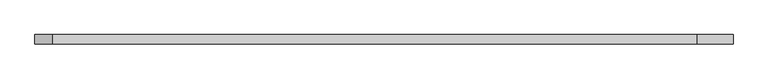
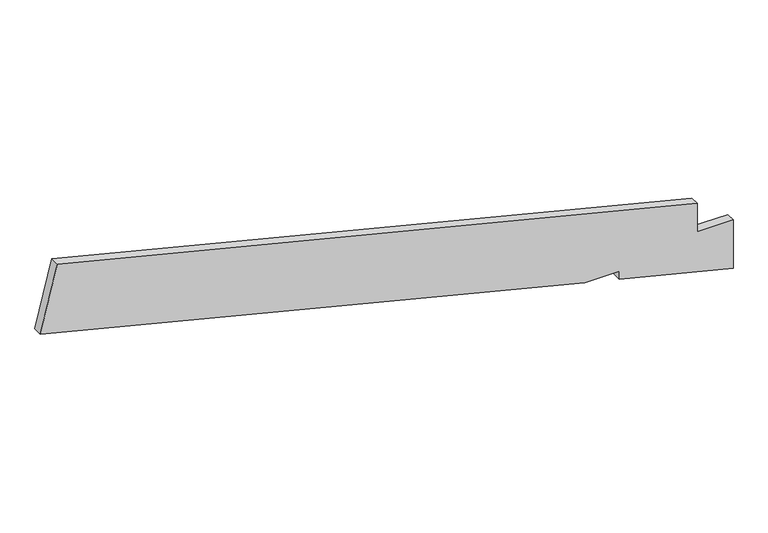
"""IFC4 building model written with IfcOpenShell, lengths in millimetres: proxy geometry, Generic Models 288:Generic Models 288:157157 : Generic Models 288:Generic Models 288:157157."""

from ifc_helpers import new_model, si_unit, frame, origin, place, context, project, spatial, polyline, outline, extrude, source, transform, mapped, element, save


def generic_models_c55f884c(model_context):
    return source(origin(), model_context, "Body", "SweptSolid", [
        extrude(outline(polyline([(6276.29133, 1895.353213), (6398.3811811, 1895.353213), (7049.7914812, -710.2879874), (6772.5732618, -779.5925423), (6218.1368229, 1438.153213), (6218.1368229, 1577.853213), (6183.2118229, 1577.853213), (6067.3243229, 2041.403213), (6276.29133, 2041.403213), (6276.29133, 1895.353213)])), frame((0.0, 5598.1378092, 0.0), z_axis=(0.0, 1.0, 0.0), x_axis=(0.0, 0.0, 1.0)), (0.0, 0.0, 1.0), 38.1),
    ])


if __name__ == "__main__":
    model = new_model("IFC4")
    model_context = context("Model", 3, world=origin())
    ifc_project = project(units=[si_unit("LENGTHUNIT", "METRE", prefix="MILLI")], contexts=[model_context])
    site = spatial("IfcSite", under=ifc_project)
    building = spatial("IfcBuilding", under=site)
    placement = place(None, origin())
    generic_models_shape = generic_models_c55f884c(model_context)
    element("IfcBuildingElementProxy", 1, Name="Generic Models 288:Generic Models 288:157157 : Generic Models 288:Generic Models 288:157157", ObjectType="Generic Models 288:Generic Models 288:157157 : Generic Models 288:Generic Models 288:157157", at=placement, inside=building, context=model_context, shape_type="MappedRepresentation", body=[
        mapped(generic_models_shape, transform((0.0, 0.0, 0.0), x_axis=(1.0, 0.0, 0.0), y_axis=(0.0, 1.0, 0.0), z_axis=(0.0, 0.0, 1.0))),
    ])
    save(model, "model.ifc")

# Revit data of these elements
# Type "Generic Models 288:Generic Models 288:157157 : Generic Models 288:Generic Models 288:157157"
#   NameOverride = "Generic Models 288:Generic Models 288:157157"
#   ObjectTypeOverride = "Generic Models 288:Generic Models 288"
#   Reference = "Generic Models 288"
#   Category = "Generic Models"
#   Tag = "157157"
# Element 1 (IfcBuildingElementProxy, "Generic Models 288:Generic Models 288:157157 : Generic Models 288:Generic Models 288:157157")
#   Materials on its faces: "_STRUCTURAL MEMBER (SEE STRUCT. DWGS) 154"
# Materials
#   "_STRUCTURAL MEMBER (SEE STRUCT. DWGS) 154": class "Unassigned", colour RGB 209 182 141, transparency 0
